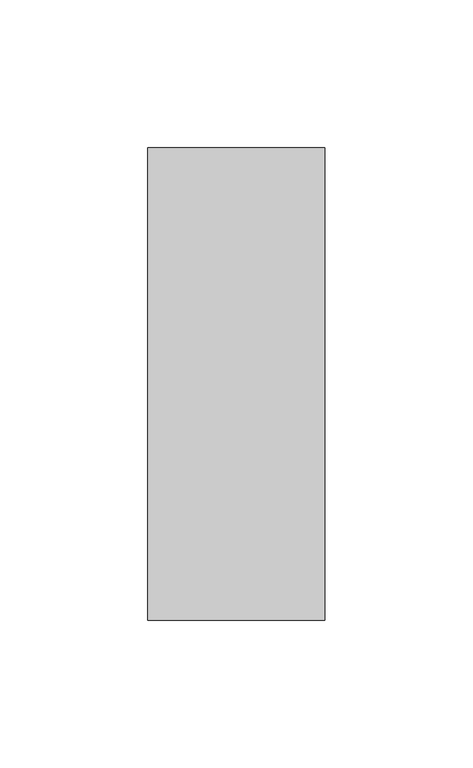
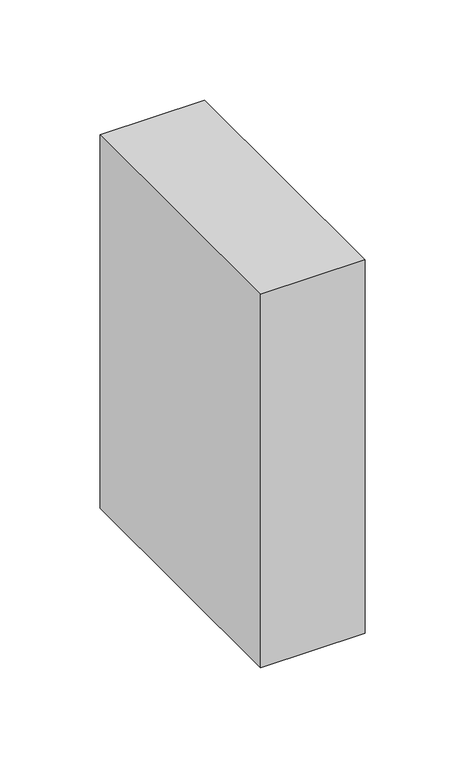
"""IFC4 building model written with IfcOpenShell, lengths in millimetres: column geometry, Madeira de lei-Coluna : Pontalete 6X16cm."""

from ifc_helpers import new_model, si_unit, frame, origin, place, context, project, spatial, polyline, outline, extrude, source, transform, mapped, element, save


def column_42eef9f8(model_context):
    return source(origin(), model_context, "Body", "SweptSolid", [
        extrude(outline(polyline([(30.0, 80.0), (30.0, -80.0), (-30.0, -80.0), (-30.0, 80.0), (30.0, 80.0)])), frame((0.0, 0.0, 6710.0), z_axis=(0.0, 0.0, 1.0), x_axis=(1.0, 0.0, 0.0)), (0.0, 0.0, 1.0), 227.1),
    ])


if __name__ == "__main__":
    model = new_model("IFC4")
    model_context = context("Model", 3, world=origin())
    ifc_project = project(units=[si_unit("LENGTHUNIT", "METRE", prefix="MILLI")], contexts=[model_context])
    site = spatial("IfcSite", under=ifc_project)
    building = spatial("IfcBuilding", under=site)
    placement = place(None, origin())
    column_shape = column_42eef9f8(model_context)
    element("IfcColumn", 1, ObjectType="Madeira de lei-Coluna : Pontalete 6X16cm", at=placement, inside=building, context=model_context, shape_type="MappedRepresentation", body=[
        mapped(column_shape, transform((0.0, 0.0, 0.0), x_axis=(1.0, 0.0, 0.0), y_axis=(0.0, 1.0, 0.0), z_axis=(0.0, 0.0, 1.0))),
    ])
    save(model, "model.ifc")

# Revit data of these elements
# Type "Madeira de lei-Coluna : Pontalete 6X16cm"
#   A = 0.01952 m²
#   b = 0.06 m
#   d = 0.16 m
#   Structural Material [instance default] = none
#   Assembly Code = ""
# Element 1 (IfcColumn, "Madeira de lei-Coluna : Pontalete 6X16cm")
#   Structural Material = .MADEIRAMENTO
#   Materials on its faces: ".MADEIRAMENTO"
# Materials
#   ".MADEIRAMENTO": class ".CC_MADEIRAS", colour RGB 212 179 113, transparency 0, Cost = 0
